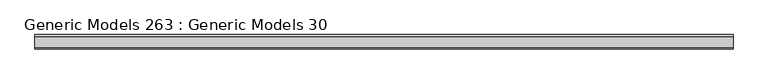
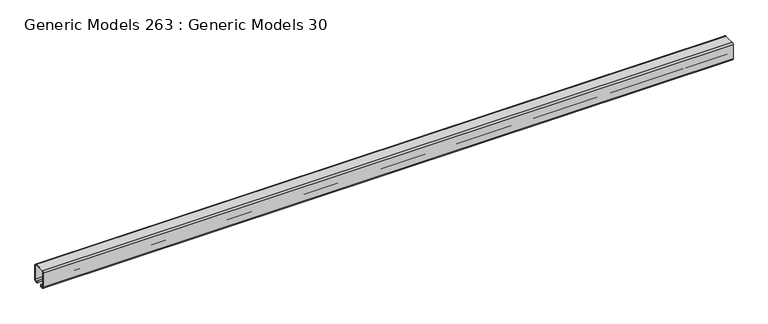
"""IFC4 building model written with IfcOpenShell, lengths in millimetres: proxy geometry, Generic Models 263 : Generic Models 30."""

from ifc_helpers import new_model, si_unit, point, frame, frame_2d, origin, place, context, project, spatial, polyline, circle_curve, trimmed, segment, composite_curve, outline, extrude, source, transform, mapped, element, save


def generic_models_263_generic_models_30_b73c1af2(model_context):
    return source(origin(), model_context, "Body", "SweptSolid", [
        extrude(outline(composite_curve([segment(polyline([(-3828.1517731, 4754.08795), (-3793.0997731, 4754.08795)]), True, "CONTINUOUS"), segment(trimmed(circle_curve(frame_2d((-3793.0997731, 4747.73795)), 6.35), [point((-3793.0997731, 4754.08795))], [point((-3786.7497731, 4747.73795))], False, "CARTESIAN"), True, "CONTINUOUS"), segment(polyline([(-3786.7497731, 4747.73795), (-3786.7497731, 4699.47795)]), True, "CONTINUOUS"), segment(trimmed(circle_curve(frame_2d((-3793.0997731, 4699.47795)), 6.35), [point((-3786.7497731, 4699.47795))], [point((-3793.0997731, 4693.12795))], False, "CARTESIAN"), True, "CONTINUOUS"), segment(polyline([(-3793.0997731, 4693.12795), (-3798.5084583, 4693.12795)]), True, "CONTINUOUS"), segment(trimmed(circle_curve(frame_2d((-3798.5084583, 4694.71545)), 1.5875), [point((-3798.5084583, 4693.12795))], [point((-3800.0667915, 4694.4125407))], False, "CARTESIAN"), True, "CONTINUOUS"), segment(polyline([(-3800.0667915, 4694.4125407), (-3801.4923072, 4701.7461831), (-3799.9761702, 4701.7461831), (-3798.590248, 4694.6162312), (-3793.0997731, 4694.6162312)]), True, "CONTINUOUS"), segment(trimmed(circle_curve(frame_2d((-3793.0997731, 4699.47795)), 4.8617188), [point((-3793.0997731, 4694.6162312))], [point((-3788.2380543, 4699.47795))], True, "CARTESIAN"), True, "CONTINUOUS"), segment(polyline([(-3788.2380543, 4699.47795), (-3788.2380543, 4747.73795)]), True, "CONTINUOUS"), segment(trimmed(circle_curve(frame_2d((-3793.0997731, 4747.73795)), 4.8617188), [point((-3788.2380543, 4747.73795))], [point((-3793.0997731, 4752.5996687))], True, "CARTESIAN"), True, "CONTINUOUS"), segment(polyline([(-3793.0997731, 4752.5996687), (-3828.1517731, 4752.5996687)]), True, "CONTINUOUS"), segment(trimmed(circle_curve(frame_2d((-3828.1517731, 4747.73795)), 4.8617188), [point((-3828.1517731, 4752.5996687))], [point((-3833.0134918, 4747.73795))], True, "CARTESIAN"), True, "CONTINUOUS"), segment(polyline([(-3833.0134918, 4747.73795), (-3833.0134918, 4699.47795)]), True, "CONTINUOUS"), segment(trimmed(circle_curve(frame_2d((-3828.1517731, 4699.47795)), 4.8617188), [point((-3833.0134918, 4699.47795))], [point((-3828.1517731, 4694.6162312))], True, "CARTESIAN"), True, "CONTINUOUS"), segment(polyline([(-3828.1517731, 4694.6162312), (-3822.6612982, 4694.6162312), (-3821.2753759, 4701.7461831), (-3819.759239, 4701.7461831), (-3821.1847546, 4694.4125407)]), True, "CONTINUOUS"), segment(trimmed(circle_curve(frame_2d((-3822.7430878, 4694.71545)), 1.5875), [point((-3821.1847546, 4694.4125407))], [point((-3822.7430878, 4693.12795))], False, "CARTESIAN"), True, "CONTINUOUS"), segment(polyline([(-3822.7430878, 4693.12795), (-3828.1517731, 4693.12795)]), True, "CONTINUOUS"), segment(trimmed(circle_curve(frame_2d((-3828.1517731, 4699.47795)), 6.35), [point((-3828.1517731, 4693.12795))], [point((-3834.5017731, 4699.47795))], False, "CARTESIAN"), True, "CONTINUOUS"), segment(polyline([(-3834.5017731, 4699.47795), (-3834.5017731, 4747.73795)]), True, "CONTINUOUS"), segment(trimmed(circle_curve(frame_2d((-3828.1517731, 4747.73795)), 6.35), [point((-3834.5017731, 4747.73795))], [point((-3828.1517731, 4754.08795))], False, "CARTESIAN"), True, "CONTINUOUS")], self_intersect=False)), frame((20327.1370052, 0.0, 0.0), z_axis=(1.0, 0.0, 0.0), x_axis=(0.0, 1.0, 0.0)), (0.0, 0.0, 1.0), 2286.0),
    ])


if __name__ == "__main__":
    model = new_model("IFC4")
    model_context = context("Model", 3, world=origin())
    ifc_project = project(units=[si_unit("LENGTHUNIT", "METRE", prefix="MILLI")], contexts=[model_context])
    site = spatial("IfcSite", under=ifc_project)
    building = spatial("IfcBuilding", under=site)
    placement = place(None, origin())
    generic_models_263_generic_models_30_shape = generic_models_263_generic_models_30_b73c1af2(model_context)
    element("IfcBuildingElementProxy", 1, Name="Generic Models 263 : Generic Models 30", ObjectType="Generic Models 263 : Generic Models 30", at=placement, inside=building, context=model_context, shape_type="MappedRepresentation", body=[
        mapped(generic_models_263_generic_models_30_shape, transform((0.0, 0.0, 0.0), x_axis=(1.0, 0.0, 0.0), y_axis=(0.0, 1.0, 0.0), z_axis=(0.0, 0.0, 1.0))),
    ])
    save(model, "model.ifc")

# Revit data of these elements
# Element 1 (IfcBuildingElementProxy, "Generic Models 263 : Generic Models 30")
#   Materials on its faces: "GALV. BOX RAIL"
# Materials
#   "GALV. BOX RAIL": class "Generic", colour RGB 212 212 212, transparency 0, Cost = 0
